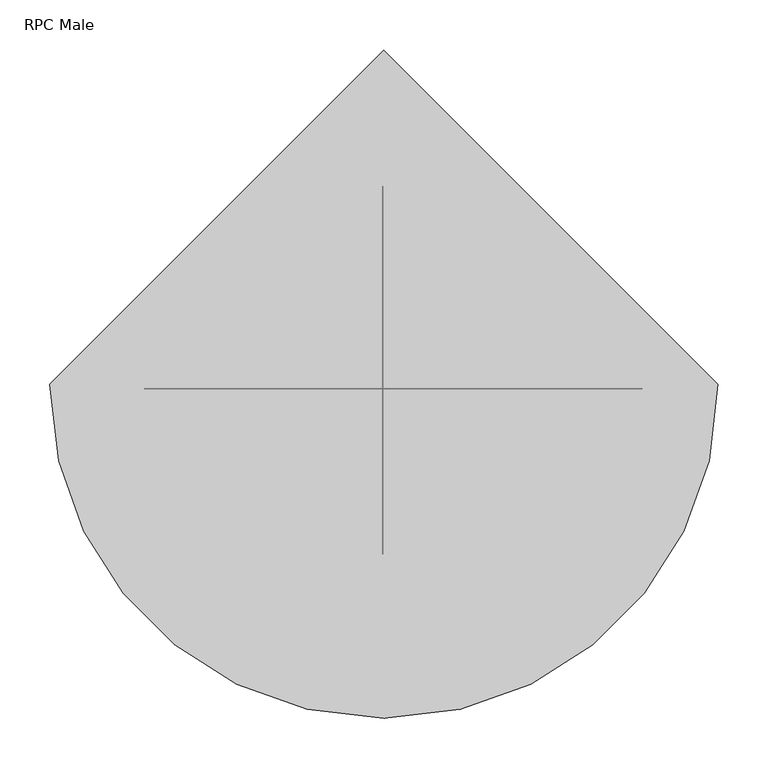
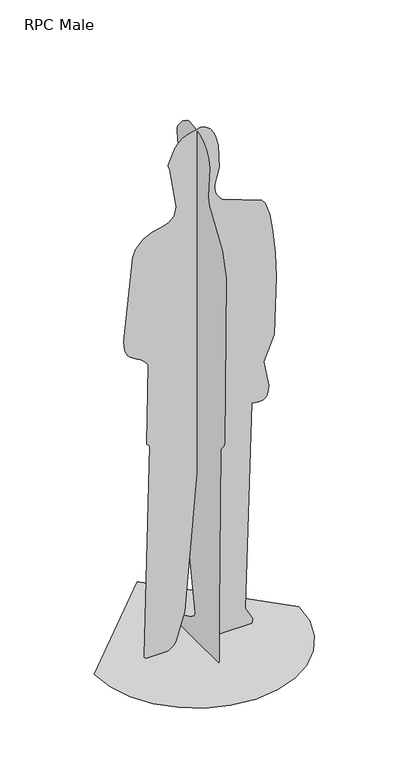
"""IFC4 building model written with IfcOpenShell, lengths in millimetres: proxy geometry, RPC Male : Dwayne."""

from ifc_helpers import new_model, si_unit, origin, place, context, project, spatial, triangles, source, transform, mapped, element, save


def rpc_male_e00c4429(model_context):
    return source(origin(), model_context, "Body", "Tessellation", [
        triangles([(-180.7519758, -4.45e-05, 5.61e-05), (-184.2427693, -8.8e-06, 2.7953145), (-186.1721755, 1.66e-05, 5.8375002), (-186.8316374, 3.35e-05, 9.127569), (-168.2846227, 8.5e-06, 733.0652109), (-173.8813015, 8.5e-06, 735.2240908), (-177.6698602, 8.1e-06, 740.93319), (-174.1985423, -8.1e-06, 1013.6682867), (-179.591309, -8.8e-06, 1024.1651751), (-188.0395216, -9.6e-06, 1032.7759867), (-198.5267085, -9.9e-06, 1040.1126028), (-210.0363257, -1.03e-05, 1046.7864687), (-221.5520472, -1.07e-05, 1053.4092476), (-232.0572199, -1.1e-05, 1060.5929661), (-240.5353907, -1.14e-05, 1068.9488514), (-245.9518842, -1.21e-05, 1078.9880642), (-249.7386988, -1.29e-05, 1091.9821838), (-252.1552483, -1.4e-05, 1106.9298906), (-253.4607645, -1.47e-05, 1122.8295742), (-224.2188539, -3.16e-05, 1405.054644), (-213.7949444, -3.31e-05, 1430.2019463), (-189.1319694, -3.46e-05, 1456.0842327), (-160.624934, -3.53e-05, 1468.8737137), (-131.9229886, -3.57e-05, 1475.6378357), (-106.6752928, -3.64e-05, 1483.4436092), (-88.5310242, -3.71e-05, 1499.3593529), (-81.1392697, -3.9e-05, 1530.4516411), (-102.942045, -4.71e-05, 1666.4696468), (-107.9472446, -4.78e-05, 1679.2650867), (-108.1474504, -4.82e-05, 1680.5741638), (-107.984815, -4.82e-05, 1682.7587688), (-107.5268306, -4.82e-05, 1685.5190655), (-106.840944, -4.86e-05, 1688.5553627), (-86.6409052, -5.11e-05, 1733.0902897), (-74.2774293, -5.19e-05, 1747.7183212), (-59.5121605, -5.26e-05, 1759.6594528), (-42.363121, -5.33e-05, 1768.7777916), (-0.9855255, -5.37e-05, 1777.9990311), (15.8808757, -5.33e-05, 1772.5528519), (29.1619555, -5.26e-05, 1761.5639877), (39.2640369, -5.19e-05, 1747.0962662), (46.5934632, -5.08e-05, 1731.2140961), (56.009163, -4.89e-05, 1695.7207684), (59.1639487, -4.41e-05, 1618.2087845), (44.4858339, -4.12e-05, 1564.7278919), (44.3096682, -4.05e-05, 1551.1862766), (46.5532813, -3.94e-05, 1537.9279289), (51.2886345, -3.86e-05, 1525.4359589), (58.5876575, -3.83e-05, 1514.1926044), (68.5223164, -3.75e-05, 1504.6808304), (198.4030241, -3.46e-05, 1454.5808361), (210.7095586, -3.38e-05, 1440.8296406), (224.9005892, -3.13e-05, 1397.8447643), (235.5369131, -2.72e-05, 1333.6069702), (242.7580384, -2.28e-05, 1256.1532677), (246.7032373, -1.77e-05, 1173.5211021), (240.2781571, -5.9e-06, 974.9290089), (206.081389, -1.1e-06, 891.6222479), (221.1961823, 4e-06, 805.6633232), (220.4650678, 5.1e-06, 788.6200321), (214.9948893, 6.3e-06, 771.8045614), (210.3552016, 6.6e-06, 765.7300776), (204.1668257, 6.6e-06, 762.0919275), (196.8959759, 7e-06, 760.3982082), (189.0090118, 7e-06, 760.1573799), (180.9721295, 7e-06, 760.8774668), (173.2515615, 6.6e-06, 762.0669291), (166.3135766, 6.6e-06, 763.2339363), (144.8011179, 4.49e-05, 59.4752896), (168.6275342, 4.74e-05, 15.3365843), (166.1985945, -4.45e-05, 5.61e-05), (66.1332089, -4.45e-05, 5.61e-05), (49.8425018, -1.03e-05, 3.9765591), (39.0246256, 1.36e-05, 14.0353), (32.5983009, 2.91e-05, 28.3297116), (-2.7441046, 9.2e-06, 720.0458748), (-54.0725034, 1.03e-05, 117.9433278), (-81.3720135, -2.13e-05, 28.0047427), (-85.5237041, -2.69e-05, 19.9172686), (-91.2433859, -3.27e-05, 12.5691172), (-99.2451413, -3.86e-05, 5.9378887), (-110.2431982, -4.45e-05, 5.61e-05), (-13.8237406, -127.6718764, 9.9621145), (-13.8237974, -127.2617633, 182.0842528), (-13.8237815, -135.2635732, 744.8695776), (-13.8237815, -136.4149928, 748.3460369), (-13.8237815, -139.3954704, 752.5736132), (-13.8237815, -143.4944026, 757.5058702), (-13.8237815, -148.0010861, 763.0962994), (-13.8237815, -152.2049901, 769.2983917), (-13.8237792, -155.3953659, 776.0656385), (-13.8237792, -156.8616281, 783.3516764), (-13.8237622, -165.9465024, 1358.6137287), (-13.8237599, -143.2743216, 1442.0927902), (-13.8237576, -71.1145501, 1552.8585583), (-13.8237576, -64.3401725, 1580.5206779), (-13.8237542, -73.5344014, 1684.7952724), (-13.8237531, -67.2131212, 1712.2161278), (-13.8237531, -55.241223, 1734.9070393), (-13.8237531, -37.9260212, 1752.7537697), (-13.8237531, -15.5748771, 1765.6426632), (-13.8237531, 11.5049084, 1773.4593372), (-13.8237531, 43.0059914, 1776.090136), (-13.8237531, 55.0860226, 1772.9164925), (-13.8237542, 79.7038559, 1756.3218658), (-13.8237554, 107.4896145, 1722.3477768), (-13.8237554, 111.5711695, 1713.01012), (-13.8237554, 112.2229284, 1702.3019073), (-13.8237588, 99.0832235, 1611.9284992), (-13.8237588, 100.6007272, 1597.8206394), (-13.8237599, 96.755177, 1579.0656796), (-13.8237622, 31.1784566, 1488.4592915), (-13.8237735, 125.7984261, 1146.7472277), (-13.8237735, 134.1993577, 1137.675107), (-13.8237747, 184.2799037, 1119.3925747), (-13.8237747, 194.4649651, 1111.9394686), (-13.8237747, 201.1343255, 1100.3801451), (-13.8237769, 203.5508567, 1084.2058416), (-13.8237769, 200.9674025, 1068.9640394), (-13.8237769, 194.2820729, 1055.8707253), (-13.8237769, 184.3928146, 1046.1415226), (-13.8237769, 172.1978105, 1040.992709), (-13.8237769, 158.595007, 1041.6399078), (-13.8237769, 144.48246, 1049.299106), (-13.8237838, 123.0429529, 785.7648285), (-13.823786, 116.906318, 707.2429499), (-13.8237928, 10.2023683, 90.6853168), (-13.823794, 17.983895, 76.1481908), (-13.8237951, 35.4714404, 63.806743), (-13.8238042, 104.5965316, 31.8661463), (-13.8238053, 119.3344402, 20.2173661), (-13.8238076, 122.9915025, 6.7192091), (-13.8238042, 122.0607091, 4.3674998), (-13.8237894, 120.3451706, 2.3141478), (-13.8237724, 119.1853577, 1.4285653), (-13.8237474, 117.8199432, 0.6534771), (-13.8237099, 116.2458387, 5.61e-05), (-13.8237077, -124.501612, 0.0), (-348.4734607, 4.7230039, 0.0001684), (-339.5987117, -72.1961519, 0.0001684), (-314.3237646, -142.8340959, 5.61e-05), (-274.6722241, -205.1669827, 5.61e-05), (-222.6681673, -257.171094, 5.61e-05), (-160.3352533, -296.8225073, 5.61e-05), (-89.6973139, -322.097527, 5.61e-05), (-12.7781649, -330.972276, 5.61e-05), (64.1409886, -322.0975634, 5.61e-05), (134.7789371, -296.8225618, 5.61e-05), (197.1118239, -257.1710577, 5.61e-05), (249.1159897, -205.1670008, 5.61e-05), (288.7673667, -142.8340595, 5.61e-05), (314.0423864, -72.1960974, 0.0001684), (322.9171354, 4.7230331, 0.0001684), (-12.7782239, 340.4182474, 0.0001684)], [[70, 71, 72], [69, 70, 72], [69, 72, 73], [69, 73, 74], [69, 74, 75], [69, 75, 76], [68, 69, 76], [82, 1, 2], [82, 2, 3], [82, 3, 4], [81, 82, 4], [80, 81, 4], [79, 80, 4], [78, 79, 4], [77, 78, 4], [77, 4, 5], [76, 77, 5], [5, 6, 7], [76, 5, 7], [76, 7, 8], [68, 76, 8], [67, 68, 8], [66, 67, 8], [65, 66, 8], [64, 65, 8], [63, 64, 8], [62, 63, 8], [61, 62, 8], [60, 61, 8], [59, 60, 8], [58, 59, 8], [57, 58, 8], [56, 57, 8], [56, 8, 9], [55, 56, 9], [55, 9, 10], [54, 55, 10], [54, 10, 11], [53, 54, 11], [53, 11, 12], [52, 53, 12], [51, 52, 12], [50, 51, 12], [50, 12, 13], [50, 13, 14], [50, 14, 15], [50, 15, 16], [50, 16, 17], [50, 17, 18], [50, 18, 19], [50, 19, 20], [50, 20, 21], [50, 21, 22], [50, 22, 23], [50, 23, 24], [50, 24, 25], [50, 25, 26], [49, 50, 26], [48, 49, 26], [48, 26, 27], [47, 48, 27], [46, 47, 27], [45, 46, 27], [44, 45, 27], [44, 27, 28], [43, 44, 28], [42, 43, 28], [42, 28, 29], [42, 29, 30], [42, 30, 31], [42, 31, 32], [42, 32, 33], [42, 33, 34], [42, 34, 35], [42, 35, 36], [42, 36, 37], [41, 42, 37], [40, 41, 37], [40, 37, 38], [40, 38, 39], [137, 138, 83], [137, 83, 84], [136, 137, 84], [135, 136, 84], [130, 131, 132], [130, 132, 133], [130, 133, 134], [130, 134, 135], [122, 123, 124], [121, 122, 124], [120, 121, 124], [119, 120, 124], [118, 119, 124], [117, 118, 124], [116, 117, 124], [115, 116, 124], [114, 115, 124], [113, 114, 124], [106, 107, 108], [105, 106, 108], [104, 105, 108], [103, 104, 108], [102, 103, 108], [101, 102, 108], [100, 101, 108], [99, 100, 108], [98, 99, 108], [97, 98, 108], [97, 108, 109], [97, 109, 110], [97, 110, 111], [96, 97, 111], [95, 96, 111], [95, 111, 112], [94, 95, 112], [93, 94, 112], [93, 112, 113], [92, 93, 113], [92, 113, 124], [92, 124, 125], [91, 92, 125], [90, 91, 125], [89, 90, 125], [88, 89, 125], [87, 88, 125], [86, 87, 125], [86, 125, 126], [85, 86, 126], [85, 126, 127], [84, 85, 127], [84, 127, 128], [135, 84, 128], [135, 128, 129], [130, 135, 129], [153, 154, 139], [152, 153, 139], [152, 139, 140], [151, 152, 140], [151, 140, 141], [151, 141, 142], [150, 151, 142], [149, 150, 142], [149, 142, 143], [149, 143, 144], [149, 144, 145], [149, 145, 146], [149, 146, 147], [149, 147, 148]], closed=False),
    ])


if __name__ == "__main__":
    model = new_model("IFC4")
    model_context = context("Model", 3, world=origin())
    ifc_project = project(units=[si_unit("LENGTHUNIT", "METRE", prefix="MILLI")], contexts=[model_context])
    site = spatial("IfcSite", under=ifc_project)
    building = spatial("IfcBuilding", under=site)
    placement = place(None, origin())
    rpc_male_shape = rpc_male_e00c4429(model_context)
    element("IfcBuildingElementProxy", 1, Name="RPC Male : Dwayne", ObjectType="RPC Male : Dwayne", at=placement, inside=building, context=model_context, shape_type="MappedRepresentation", body=[
        mapped(rpc_male_shape, transform((0.0, 0.0, 0.0), x_axis=(1.0, 0.0, 0.0), y_axis=(0.0, 1.0, 0.0), z_axis=(0.0, 0.0, 1.0))),
    ])
    save(model, "model.ifc")

# Revit data of these elements
# Type "RPC Male : Dwayne"
#   built-in parameter 1005198 = "{2, 15},{22, RPC-8-G1AE-S4G0-CKUK-A},{1, 0},{1, 0},{2, 15},{1, 8},{5, Color},{1, 0},{1, 0},{3, 0.8},{3, 0.8},{3, 0.8},{1, 8},{7, BBoxMin},{1, 0},{1, 0},{1, 0},{1, 0},{1, 0},{1, 8},{7, BBoxMax},{1, 0},{1, 0},{1, 0},{1, 0},{1, 0},{2, 11},{9, RPCTypeId},{1, 0},{1, 0},{22, RPC-8-G1AE-S4G0-CKUK-A},{1, 6},{14, RPCPlantHeight},{1, 0},{1, 0},{7, 5.83333},{2, 11},{7, keyword},{1, 0},{1, 0},{45, :RPCs:People [Business-Hispanic]:Geometry:RPC},{2, 11},{8, category},{1, 0},{1, 0},{26, People [Business-Hispanic]},{2, 11},{12, LocalizedUID},{1, 0},{1, 0},{6, Dwayne},{2, 14},{6, Height},{1, 0},{1, 0},{7, 5.83333},{1, 2},{16, Cast Reflections},{1, 0},{1, 0},{1, 0},{1, 2},{6, Jitter},{1, 0},{1, 0},{1, 1},{1, 2},{9, Billboard},{1, 0},{1, 0},{1, 0},{1, 2},{12, Cast Shadows},{1, 0},{1, 0},{1, 1},{1, 2},{20, Apply Filter Effects},{1, 0},{1, 0},{1, 0},{2, 11},{28, Apply Filter Effects-Text-FC},{1, 0},{1, 0},{4, None},{21, assetlibrary_base.fbx},{1, 5},"
#   built-in parameter 1005195 = "RPC-8-G1AE-S4G0-CKUK-A"
#   Height = 0
